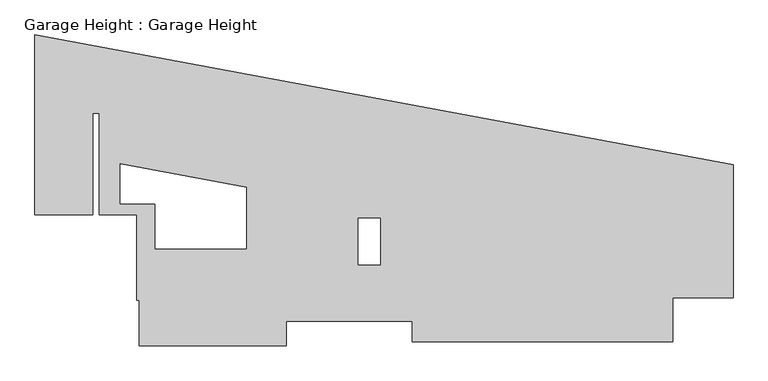
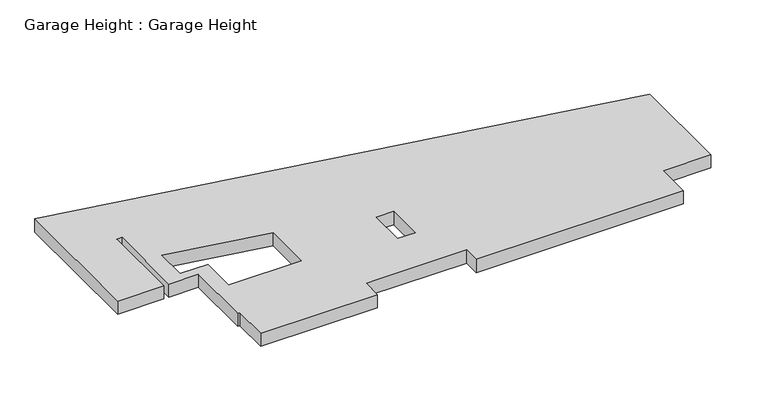
"""IFC4 building model written with IfcOpenShell, lengths in millimetres: proxy geometry, Garage Height : Garage Height."""

from ifc_helpers import new_model, si_unit, frame, origin, place, context, project, spatial, polyline, outline, extrude, source, transform, mapped, element, save


def garage_height_garage_height_b4313ec3(model_context):
    return source(origin(), model_context, "Body", "SweptSolid", [
        extrude(outline(polyline([(3.175, 21841.6157788), (3.175, 5638.8), (-7340.6, 5638.8), (-7340.6, 255.042208), (-39065.2, 255.042208), (-39065.2, 2768.6), (-54457.6, 2768.6), (-54457.6, -228.6), (-72348.677375, -228.6), (-72348.677375, 5283.2), (-72669.4, 5283.2), (-72669.4, 15697.2), (-77190.6, 15697.2), (-77190.6, 28117.8), (-78016.1, 28117.8), (-78016.1, 15697.2), (-85051.9, 15697.2), (-85051.9, 37634.7127261), (3.175, 21841.6157788)]), holes=[polyline([(-59283.6, 19075.3995851), (-74676.0, 21944.8881192), (-74676.0, 17094.1995851), (-70384.2397499, 17094.1995851), (-70384.2397499, 11607.8), (-59283.6, 11607.8), (-59283.6, 19075.3995851)]), polyline([(-42951.4, 9664.7), (-42951.4, 15316.2), (-45669.2, 15316.2), (-45669.2, 9664.7), (-42951.4, 9664.7)])]), frame((0.0, 0.0, 9366.25), z_axis=(0.0, 0.0, 1.0), x_axis=(1.0, 0.0, 0.0)), (0.0, 0.0, 1.0), 2133.6),
    ])


if __name__ == "__main__":
    model = new_model("IFC4")
    model_context = context("Model", 3, world=origin())
    ifc_project = project(units=[si_unit("LENGTHUNIT", "METRE", prefix="MILLI")], contexts=[model_context])
    site = spatial("IfcSite", under=ifc_project)
    building = spatial("IfcBuilding", under=site)
    placement = place(None, origin())
    garage_height_garage_height_shape = garage_height_garage_height_b4313ec3(model_context)
    element("IfcBuildingElementProxy", 1, Name="Garage Height : Garage Height", ObjectType="Garage Height : Garage Height", at=placement, inside=building, context=model_context, shape_type="MappedRepresentation", body=[
        mapped(garage_height_garage_height_shape, transform((0.0, 0.0, 0.0), x_axis=(1.0, 0.0, 0.0), y_axis=(0.0, 1.0, 0.0), z_axis=(0.0, 0.0, 1.0))),
    ])
    save(model, "model.ifc")

# Revit data of these elements
# Element 1 (IfcBuildingElementProxy, "Garage Height : Garage Height")
#   Materials on its faces: "Lower Parking Clearance Zone"
# Materials
#   "Lower Parking Clearance Zone": class "Generic", colour RGB 255 0 0, transparency 0, Cost = 0
